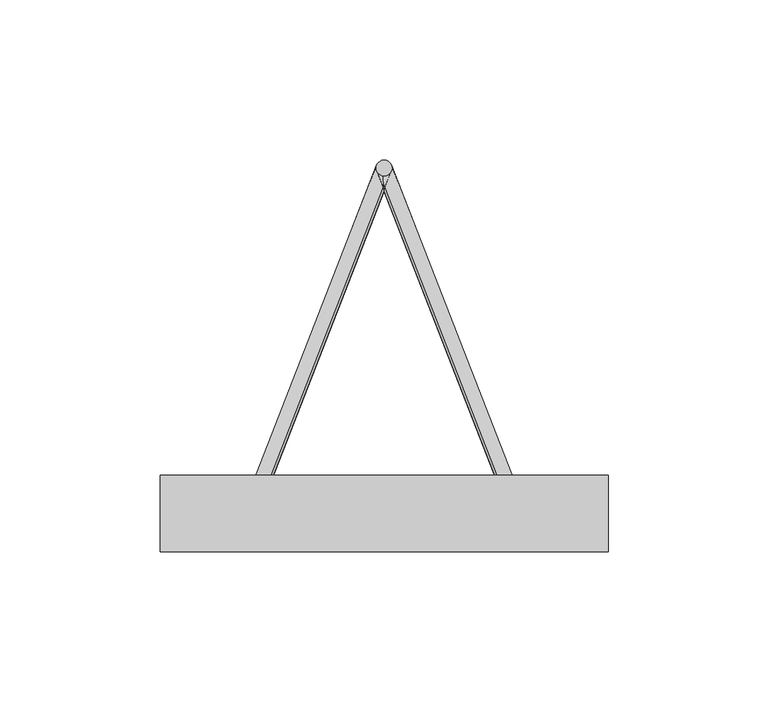
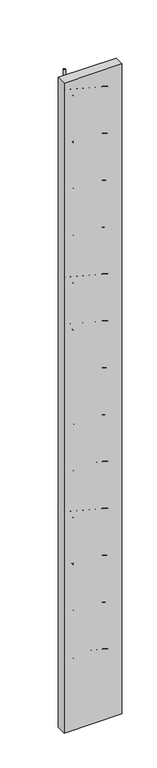
"""IFC4 building model written with IfcOpenShell, lengths in millimetres: proxy geometry, Vigota 2 (Pano 8) (Mf = 158)."""

from ifc_helpers import new_model, si_unit, point, frame, frame_2d, origin, origin_with_axes, origin_2d, place, context, project, spatial, polyline, circle_curve, trimmed, segment, composite_curve, outline, extrude, source, transform, mapped, element, save


def structural_framing_ade8639b(model_context):
    return source(origin(), model_context, "Body", "SweptSolid", [
        extrude(outline(polyline([(-70.0, 12.0), (70.0, 12.0), (70.0, -12.0), (-70.0, -12.0), (-70.0, 12.0)])), origin_with_axes(), (0.0, 0.0, 1.0), 1663.655183),
        extrude(outline(composite_curve([segment(trimmed(circle_curve(frame_2d((42.0, 0.0)), 2.5), [point((44.5, 0.0))], [point((39.5, 0.0))], False, "CARTESIAN"), True, "CONTINUOUS"), segment(trimmed(circle_curve(frame_2d((42.0, 0.0)), 2.5), [point((39.5, 0.0))], [point((44.5, 0.0))], False, "CARTESIAN"), True, "CONTINUOUS")], self_intersect=False)), frame((0.0, 0.0, 28.0), z_axis=(0.0, 0.0, 1.0), x_axis=(1.0, 0.0, 0.0)), (0.0, 0.0, 1.0), 1607.655183),
        extrude(outline(composite_curve([segment(trimmed(circle_curve(frame_2d((0.0, 108.0)), 2.5), [point((2.5, 108.0))], [point((-2.5, 108.0))], False, "CARTESIAN"), True, "CONTINUOUS"), segment(trimmed(circle_curve(frame_2d((0.0, 108.0)), 2.5), [point((-2.5, 108.0))], [point((2.5, 108.0))], False, "CARTESIAN"), True, "CONTINUOUS")], self_intersect=False)), frame((0.0, 0.0, 61.8275917), z_axis=(0.0, 0.0, 1.0), x_axis=(1.0, 0.0, 0.0)), (0.0, 0.0, 1.0), 1540.0),
        extrude(outline(composite_curve([segment(trimmed(circle_curve(origin_2d(), 2.5), [point((2.5, 0.0))], [point((-2.5, 0.0))], False, "CARTESIAN"), True, "CONTINUOUS"), segment(trimmed(circle_curve(origin_2d(), 2.5), [point((-2.5, 0.0))], [point((2.5, 0.0))], False, "CARTESIAN"), True, "CONTINUOUS")], self_intersect=False)), frame((42.0, 0.0, 51.8275917), z_axis=(-0.3218603428886276, 0.8276408817707567, 0.4598004898837537), x_axis=(0.8192319205108605, -3.936835275445103e-11, 0.5734623443750141)), (0.0, 0.0, 1.0), 130.491379),
        extrude(outline(composite_curve([segment(trimmed(circle_curve(origin_2d(), 2.5), [point((2.5, 0.0))], [point((-2.5, 0.0))], False, "CARTESIAN"), True, "CONTINUOUS"), segment(trimmed(circle_curve(origin_2d(), 2.5), [point((-2.5, 0.0))], [point((2.5, 0.0))], False, "CARTESIAN"), True, "CONTINUOUS")], self_intersect=False)), frame((0.0, 108.0, 111.8275917), z_axis=(0.3218603428886276, -0.8276408817707567, 0.4598004898837537), x_axis=(0.8192319205108605, -3.936835275445103e-11, -0.5734623443750141)), (0.0, 0.0, 1.0), 130.491379),
        extrude(outline(composite_curve([segment(trimmed(circle_curve(origin_2d(), 2.5), [point((2.5, 0.0))], [point((-2.5, 0.0))], False, "CARTESIAN"), True, "CONTINUOUS"), segment(trimmed(circle_curve(origin_2d(), 2.5), [point((-2.5, 0.0))], [point((2.5, 0.0))], False, "CARTESIAN"), True, "CONTINUOUS")], self_intersect=False)), frame((42.0, 0.0, 171.8275917), z_axis=(-0.3218603428886276, 0.8276408817707567, 0.4598004898837537), x_axis=(0.8192319205108605, -3.936835275445103e-11, 0.5734623443750141)), (0.0, 0.0, 1.0), 130.491379),
        extrude(outline(composite_curve([segment(trimmed(circle_curve(origin_2d(), 2.5), [point((2.5, 0.0))], [point((-2.5, 0.0))], False, "CARTESIAN"), True, "CONTINUOUS"), segment(trimmed(circle_curve(origin_2d(), 2.5), [point((-2.5, 0.0))], [point((2.5, 0.0))], False, "CARTESIAN"), True, "CONTINUOUS")], self_intersect=False)), frame((0.0, 108.0, 231.8275917), z_axis=(0.3218603428886276, -0.8276408817707567, 0.4598004898837537), x_axis=(0.8192319205108605, -3.936835275445103e-11, -0.5734623443750141)), (0.0, 0.0, 1.0), 130.491379),
        extrude(outline(composite_curve([segment(trimmed(circle_curve(origin_2d(), 2.5), [point((2.5, 0.0))], [point((-2.5, 0.0))], False, "CARTESIAN"), True, "CONTINUOUS"), segment(trimmed(circle_curve(origin_2d(), 2.5), [point((-2.5, 0.0))], [point((2.5, 0.0))], False, "CARTESIAN"), True, "CONTINUOUS")], self_intersect=False)), frame((42.0, 0.0, 291.8275917), z_axis=(-0.3218603428886276, 0.8276408817707567, 0.4598004898837537), x_axis=(0.8192319205108605, -3.936835275445103e-11, 0.5734623443750141)), (0.0, 0.0, 1.0), 130.491379),
        extrude(outline(composite_curve([segment(trimmed(circle_curve(origin_2d(), 2.5), [point((2.5, 0.0))], [point((-2.5, 0.0))], False, "CARTESIAN"), True, "CONTINUOUS"), segment(trimmed(circle_curve(origin_2d(), 2.5), [point((-2.5, 0.0))], [point((2.5, 0.0))], False, "CARTESIAN"), True, "CONTINUOUS")], self_intersect=False)), frame((0.0, 108.0, 351.8275917), z_axis=(0.3218603428886276, -0.8276408817707567, 0.4598004898837537), x_axis=(0.8192319205108605, -3.936835275445103e-11, -0.5734623443750141)), (0.0, 0.0, 1.0), 130.491379),
        extrude(outline(composite_curve([segment(trimmed(circle_curve(origin_2d(), 2.5), [point((2.5, 0.0))], [point((-2.5, 0.0))], False, "CARTESIAN"), True, "CONTINUOUS"), segment(trimmed(circle_curve(origin_2d(), 2.5), [point((-2.5, 0.0))], [point((2.5, 0.0))], False, "CARTESIAN"), True, "CONTINUOUS")], self_intersect=False)), frame((42.0, 0.0, 411.8275917), z_axis=(-0.3218603428886276, 0.8276408817707567, 0.4598004898837537), x_axis=(0.8192319205108605, -3.936835275445103e-11, 0.5734623443750141)), (0.0, 0.0, 1.0), 130.491379),
        extrude(outline(composite_curve([segment(trimmed(circle_curve(origin_2d(), 2.5), [point((2.5, 0.0))], [point((-2.5, 0.0))], False, "CARTESIAN"), True, "CONTINUOUS"), segment(trimmed(circle_curve(origin_2d(), 2.5), [point((-2.5, 0.0))], [point((2.5, 0.0))], False, "CARTESIAN"), True, "CONTINUOUS")], self_intersect=False)), frame((0.0, 108.0, 471.8275917), z_axis=(0.3218603428886276, -0.8276408817707567, 0.4598004898837537), x_axis=(0.8192319205108605, -3.936835275445103e-11, -0.5734623443750141)), (0.0, 0.0, 1.0), 130.491379),
        extrude(outline(composite_curve([segment(trimmed(circle_curve(origin_2d(), 2.5), [point((2.5, 0.0))], [point((-2.5, 0.0))], False, "CARTESIAN"), True, "CONTINUOUS"), segment(trimmed(circle_curve(origin_2d(), 2.5), [point((-2.5, 0.0))], [point((2.5, 0.0))], False, "CARTESIAN"), True, "CONTINUOUS")], self_intersect=False)), frame((42.0, 0.0, 531.8275917), z_axis=(-0.3218603428886276, 0.8276408817707567, 0.4598004898837537), x_axis=(0.8192319205108605, -3.936835275445103e-11, 0.5734623443750141)), (0.0, 0.0, 1.0), 130.491379),
        extrude(outline(composite_curve([segment(trimmed(circle_curve(origin_2d(), 2.5), [point((2.5, 0.0))], [point((-2.5, 0.0))], False, "CARTESIAN"), True, "CONTINUOUS"), segment(trimmed(circle_curve(origin_2d(), 2.5), [point((-2.5, 0.0))], [point((2.5, 0.0))], False, "CARTESIAN"), True, "CONTINUOUS")], self_intersect=False)), frame((0.0, 108.0, 591.8275917), z_axis=(0.3218603428886276, -0.8276408817707567, 0.4598004898837537), x_axis=(0.8192319205108605, -3.936835275445103e-11, -0.5734623443750141)), (0.0, 0.0, 1.0), 130.491379),
        extrude(outline(composite_curve([segment(trimmed(circle_curve(origin_2d(), 2.5), [point((2.5, 0.0))], [point((-2.5, 0.0))], False, "CARTESIAN"), True, "CONTINUOUS"), segment(trimmed(circle_curve(origin_2d(), 2.5), [point((-2.5, 0.0))], [point((2.5, 0.0))], False, "CARTESIAN"), True, "CONTINUOUS")], self_intersect=False)), frame((42.0, 0.0, 651.8275917), z_axis=(-0.3218603428886276, 0.8276408817707567, 0.4598004898837537), x_axis=(0.8192319205108605, -3.936835275445103e-11, 0.5734623443750141)), (0.0, 0.0, 1.0), 130.491379),
        extrude(outline(composite_curve([segment(trimmed(circle_curve(origin_2d(), 2.5), [point((2.5, 0.0))], [point((-2.5, 0.0))], False, "CARTESIAN"), True, "CONTINUOUS"), segment(trimmed(circle_curve(origin_2d(), 2.5), [point((-2.5, 0.0))], [point((2.5, 0.0))], False, "CARTESIAN"), True, "CONTINUOUS")], self_intersect=False)), frame((0.0, 108.0, 711.8275917), z_axis=(0.3218603428886276, -0.8276408817707567, 0.4598004898837537), x_axis=(0.8192319205108605, -3.936835275445103e-11, -0.5734623443750141)), (0.0, 0.0, 1.0), 130.491379),
        extrude(outline(composite_curve([segment(trimmed(circle_curve(origin_2d(), 2.5), [point((2.5, 0.0))], [point((-2.5, 0.0))], False, "CARTESIAN"), True, "CONTINUOUS"), segment(trimmed(circle_curve(origin_2d(), 2.5), [point((-2.5, 0.0))], [point((2.5, 0.0))], False, "CARTESIAN"), True, "CONTINUOUS")], self_intersect=False)), frame((42.0, 0.0, 771.8275917), z_axis=(-0.3218603428886276, 0.8276408817707567, 0.4598004898837537), x_axis=(0.8192319205108605, -3.936835275445103e-11, 0.5734623443750141)), (0.0, 0.0, 1.0), 130.491379),
        extrude(outline(composite_curve([segment(trimmed(circle_curve(origin_2d(), 2.5), [point((2.5, 0.0))], [point((-2.5, 0.0))], False, "CARTESIAN"), True, "CONTINUOUS"), segment(trimmed(circle_curve(origin_2d(), 2.5), [point((-2.5, 0.0))], [point((2.5, 0.0))], False, "CARTESIAN"), True, "CONTINUOUS")], self_intersect=False)), frame((0.0, 108.0, 831.8275917), z_axis=(0.3218603428886276, -0.8276408817707567, 0.4598004898837537), x_axis=(0.8192319205108605, -3.936835275445103e-11, -0.5734623443750141)), (0.0, 0.0, 1.0), 130.491379),
        extrude(outline(composite_curve([segment(trimmed(circle_curve(origin_2d(), 2.5), [point((2.5, 0.0))], [point((-2.5, 0.0))], False, "CARTESIAN"), True, "CONTINUOUS"), segment(trimmed(circle_curve(origin_2d(), 2.5), [point((-2.5, 0.0))], [point((2.5, 0.0))], False, "CARTESIAN"), True, "CONTINUOUS")], self_intersect=False)), frame((42.0, 0.0, 891.8275917), z_axis=(-0.3218603428886276, 0.8276408817707567, 0.4598004898837537), x_axis=(0.8192319205108605, -3.936835275445103e-11, 0.5734623443750141)), (0.0, 0.0, 1.0), 130.491379),
        extrude(outline(composite_curve([segment(trimmed(circle_curve(origin_2d(), 2.5), [point((2.5, 0.0))], [point((-2.5, 0.0))], False, "CARTESIAN"), True, "CONTINUOUS"), segment(trimmed(circle_curve(origin_2d(), 2.5), [point((-2.5, 0.0))], [point((2.5, 0.0))], False, "CARTESIAN"), True, "CONTINUOUS")], self_intersect=False)), frame((0.0, 108.0, 951.8275917), z_axis=(0.3218603428886276, -0.8276408817707567, 0.4598004898837537), x_axis=(0.8192319205108605, -3.936835275445103e-11, -0.5734623443750141)), (0.0, 0.0, 1.0), 130.491379),
        extrude(outline(composite_curve([segment(trimmed(circle_curve(origin_2d(), 2.5), [point((2.5, 0.0))], [point((-2.5, 0.0))], False, "CARTESIAN"), True, "CONTINUOUS"), segment(trimmed(circle_curve(origin_2d(), 2.5), [point((-2.5, 0.0))], [point((2.5, 0.0))], False, "CARTESIAN"), True, "CONTINUOUS")], self_intersect=False)), frame((42.0, 0.0, 1011.8275917), z_axis=(-0.3218603428886276, 0.8276408817707567, 0.4598004898837537), x_axis=(0.8192319205108605, -3.936835275445103e-11, 0.5734623443750141)), (0.0, 0.0, 1.0), 130.491379),
        extrude(outline(composite_curve([segment(trimmed(circle_curve(origin_2d(), 2.5), [point((2.5, 0.0))], [point((-2.5, 0.0))], False, "CARTESIAN"), True, "CONTINUOUS"), segment(trimmed(circle_curve(origin_2d(), 2.5), [point((-2.5, 0.0))], [point((2.5, 0.0))], False, "CARTESIAN"), True, "CONTINUOUS")], self_intersect=False)), frame((0.0, 108.0, 1071.827592), z_axis=(0.3218603428886276, -0.8276408817707567, 0.4598004898837537), x_axis=(0.8192319205108605, -3.936835275445103e-11, -0.5734623443750141)), (0.0, 0.0, 1.0), 130.491379),
        extrude(outline(composite_curve([segment(trimmed(circle_curve(origin_2d(), 2.5), [point((2.5, 0.0))], [point((-2.5, 0.0))], False, "CARTESIAN"), True, "CONTINUOUS"), segment(trimmed(circle_curve(origin_2d(), 2.5), [point((-2.5, 0.0))], [point((2.5, 0.0))], False, "CARTESIAN"), True, "CONTINUOUS")], self_intersect=False)), frame((42.0, 0.0, 1131.827592), z_axis=(-0.3218603428886276, 0.8276408817707567, 0.4598004898837537), x_axis=(0.8192319205108605, -3.936835275445103e-11, 0.5734623443750141)), (0.0, 0.0, 1.0), 130.491379),
        extrude(outline(composite_curve([segment(trimmed(circle_curve(origin_2d(), 2.5), [point((2.5, 0.0))], [point((-2.5, 0.0))], False, "CARTESIAN"), True, "CONTINUOUS"), segment(trimmed(circle_curve(origin_2d(), 2.5), [point((-2.5, 0.0))], [point((2.5, 0.0))], False, "CARTESIAN"), True, "CONTINUOUS")], self_intersect=False)), frame((0.0, 108.0, 1191.827592), z_axis=(0.3218603428886276, -0.8276408817707567, 0.4598004898837537), x_axis=(0.8192319205108605, -3.936835275445103e-11, -0.5734623443750141)), (0.0, 0.0, 1.0), 130.491379),
        extrude(outline(composite_curve([segment(trimmed(circle_curve(origin_2d(), 2.5), [point((2.5, 0.0))], [point((-2.5, 0.0))], False, "CARTESIAN"), True, "CONTINUOUS"), segment(trimmed(circle_curve(origin_2d(), 2.5), [point((-2.5, 0.0))], [point((2.5, 0.0))], False, "CARTESIAN"), True, "CONTINUOUS")], self_intersect=False)), frame((42.0, 0.0, 1251.827592), z_axis=(-0.3218603428886276, 0.8276408817707567, 0.4598004898837537), x_axis=(0.8192319205108605, -3.936835275445103e-11, 0.5734623443750141)), (0.0, 0.0, 1.0), 130.491379),
        extrude(outline(composite_curve([segment(trimmed(circle_curve(origin_2d(), 2.5), [point((2.5, 0.0))], [point((-2.5, 0.0))], False, "CARTESIAN"), True, "CONTINUOUS"), segment(trimmed(circle_curve(origin_2d(), 2.5), [point((-2.5, 0.0))], [point((2.5, 0.0))], False, "CARTESIAN"), True, "CONTINUOUS")], self_intersect=False)), frame((0.0, 108.0, 1311.827592), z_axis=(0.3218603428886276, -0.8276408817707567, 0.4598004898837537), x_axis=(0.8192319205108605, -3.936835275445103e-11, -0.5734623443750141)), (0.0, 0.0, 1.0), 130.491379),
        extrude(outline(composite_curve([segment(trimmed(circle_curve(origin_2d(), 2.5), [point((2.5, 0.0))], [point((-2.5, 0.0))], False, "CARTESIAN"), True, "CONTINUOUS"), segment(trimmed(circle_curve(origin_2d(), 2.5), [point((-2.5, 0.0))], [point((2.5, 0.0))], False, "CARTESIAN"), True, "CONTINUOUS")], self_intersect=False)), frame((42.0, 0.0, 1371.827592), z_axis=(-0.3218603428886276, 0.8276408817707567, 0.4598004898837537), x_axis=(0.8192319205108605, -3.936835275445103e-11, 0.5734623443750141)), (0.0, 0.0, 1.0), 130.491379),
        extrude(outline(composite_curve([segment(trimmed(circle_curve(origin_2d(), 2.5), [point((2.5, 0.0))], [point((-2.5, 0.0))], False, "CARTESIAN"), True, "CONTINUOUS"), segment(trimmed(circle_curve(origin_2d(), 2.5), [point((-2.5, 0.0))], [point((2.5, 0.0))], False, "CARTESIAN"), True, "CONTINUOUS")], self_intersect=False)), frame((0.0, 108.0, 1431.827592), z_axis=(0.3218603428886276, -0.8276408817707567, 0.4598004898837537), x_axis=(0.8192319205108605, -3.936835275445103e-11, -0.5734623443750141)), (0.0, 0.0, 1.0), 130.491379),
        extrude(outline(composite_curve([segment(trimmed(circle_curve(origin_2d(), 2.5), [point((2.5, 0.0))], [point((-2.5, 0.0))], False, "CARTESIAN"), True, "CONTINUOUS"), segment(trimmed(circle_curve(origin_2d(), 2.5), [point((-2.5, 0.0))], [point((2.5, 0.0))], False, "CARTESIAN"), True, "CONTINUOUS")], self_intersect=False)), frame((42.0, 0.0, 1491.827592), z_axis=(-0.3218603428886276, 0.8276408817707567, 0.4598004898837537), x_axis=(0.8192319205108605, -3.936835275445103e-11, 0.5734623443750141)), (0.0, 0.0, 1.0), 130.491379),
        extrude(outline(composite_curve([segment(trimmed(circle_curve(origin_2d(), 2.5), [point((2.5, 0.0))], [point((-2.5, 0.0))], False, "CARTESIAN"), True, "CONTINUOUS"), segment(trimmed(circle_curve(origin_2d(), 2.5), [point((-2.5, 0.0))], [point((2.5, 0.0))], False, "CARTESIAN"), True, "CONTINUOUS")], self_intersect=False)), frame((0.0, 108.0, 1551.827592), z_axis=(0.3218603428886276, -0.8276408817707567, 0.4598004898837537), x_axis=(0.8192319205108605, -3.936835275445103e-11, -0.5734623443750141)), (0.0, 0.0, 1.0), 130.491379),
        extrude(outline(composite_curve([segment(trimmed(circle_curve(frame_2d((-42.0, 0.0)), 2.5), [point((-39.5, 0.0))], [point((-44.5, 0.0))], False, "CARTESIAN"), True, "CONTINUOUS"), segment(trimmed(circle_curve(frame_2d((-42.0, 0.0)), 2.5), [point((-44.5, 0.0))], [point((-39.5, 0.0))], False, "CARTESIAN"), True, "CONTINUOUS")], self_intersect=False)), frame((0.0, 0.0, 28.0), z_axis=(0.0, 0.0, 1.0), x_axis=(1.0, 0.0, 0.0)), (0.0, 0.0, 1.0), 1607.655183),
        extrude(outline(composite_curve([segment(trimmed(circle_curve(origin_2d(), 2.5), [point((2.5, 0.0))], [point((-2.5, 0.0))], False, "CARTESIAN"), True, "CONTINUOUS"), segment(trimmed(circle_curve(origin_2d(), 2.5), [point((-2.5, 0.0))], [point((2.5, 0.0))], False, "CARTESIAN"), True, "CONTINUOUS")], self_intersect=False)), frame((-42.0, 0.0, 51.8275917), z_axis=(0.3218603428886276, 0.8276408817707567, 0.4598004898837537), x_axis=(0.8192319205108605, 3.936835275445103e-11, -0.5734623443750141)), (0.0, 0.0, 1.0), 130.491379),
        extrude(outline(composite_curve([segment(trimmed(circle_curve(origin_2d(), 2.5), [point((2.5, 0.0))], [point((-2.5, 0.0))], False, "CARTESIAN"), True, "CONTINUOUS"), segment(trimmed(circle_curve(origin_2d(), 2.5), [point((-2.5, 0.0))], [point((2.5, 0.0))], False, "CARTESIAN"), True, "CONTINUOUS")], self_intersect=False)), frame((0.0, 108.0, 111.8275917), z_axis=(-0.3218603428886276, -0.8276408817707567, 0.4598004898837537), x_axis=(0.8192319205108605, 3.936835275445103e-11, 0.5734623443750141)), (0.0, 0.0, 1.0), 130.491379),
        extrude(outline(composite_curve([segment(trimmed(circle_curve(origin_2d(), 2.5), [point((2.5, 0.0))], [point((-2.5, 0.0))], False, "CARTESIAN"), True, "CONTINUOUS"), segment(trimmed(circle_curve(origin_2d(), 2.5), [point((-2.5, 0.0))], [point((2.5, 0.0))], False, "CARTESIAN"), True, "CONTINUOUS")], self_intersect=False)), frame((-42.0, 0.0, 171.8275917), z_axis=(0.3218603428886276, 0.8276408817707567, 0.4598004898837537), x_axis=(0.8192319205108605, 3.936835275445103e-11, -0.5734623443750141)), (0.0, 0.0, 1.0), 130.491379),
        extrude(outline(composite_curve([segment(trimmed(circle_curve(origin_2d(), 2.5), [point((2.5, 0.0))], [point((-2.5, 0.0))], False, "CARTESIAN"), True, "CONTINUOUS"), segment(trimmed(circle_curve(origin_2d(), 2.5), [point((-2.5, 0.0))], [point((2.5, 0.0))], False, "CARTESIAN"), True, "CONTINUOUS")], self_intersect=False)), frame((0.0, 108.0, 231.8275917), z_axis=(-0.3218603428886276, -0.8276408817707567, 0.4598004898837537), x_axis=(0.8192319205108605, 3.936835275445103e-11, 0.5734623443750141)), (0.0, 0.0, 1.0), 130.491379),
        extrude(outline(composite_curve([segment(trimmed(circle_curve(origin_2d(), 2.5), [point((2.5, 0.0))], [point((-2.5, 0.0))], False, "CARTESIAN"), True, "CONTINUOUS"), segment(trimmed(circle_curve(origin_2d(), 2.5), [point((-2.5, 0.0))], [point((2.5, 0.0))], False, "CARTESIAN"), True, "CONTINUOUS")], self_intersect=False)), frame((-42.0, 0.0, 291.8275917), z_axis=(0.3218603428886276, 0.8276408817707567, 0.4598004898837537), x_axis=(0.8192319205108605, 3.936835275445103e-11, -0.5734623443750141)), (0.0, 0.0, 1.0), 130.491379),
        extrude(outline(composite_curve([segment(trimmed(circle_curve(origin_2d(), 2.5), [point((2.5, 0.0))], [point((-2.5, 0.0))], False, "CARTESIAN"), True, "CONTINUOUS"), segment(trimmed(circle_curve(origin_2d(), 2.5), [point((-2.5, 0.0))], [point((2.5, 0.0))], False, "CARTESIAN"), True, "CONTINUOUS")], self_intersect=False)), frame((0.0, 108.0, 351.8275917), z_axis=(-0.3218603428886276, -0.8276408817707567, 0.4598004898837537), x_axis=(0.8192319205108605, 3.936835275445103e-11, 0.5734623443750141)), (0.0, 0.0, 1.0), 130.491379),
        extrude(outline(composite_curve([segment(trimmed(circle_curve(origin_2d(), 2.5), [point((2.5, 0.0))], [point((-2.5, 0.0))], False, "CARTESIAN"), True, "CONTINUOUS"), segment(trimmed(circle_curve(origin_2d(), 2.5), [point((-2.5, 0.0))], [point((2.5, 0.0))], False, "CARTESIAN"), True, "CONTINUOUS")], self_intersect=False)), frame((-42.0, 0.0, 411.8275917), z_axis=(0.3218603428886276, 0.8276408817707567, 0.4598004898837537), x_axis=(0.8192319205108605, 3.936835275445103e-11, -0.5734623443750141)), (0.0, 0.0, 1.0), 130.491379),
        extrude(outline(composite_curve([segment(trimmed(circle_curve(origin_2d(), 2.5), [point((2.5, 0.0))], [point((-2.5, 0.0))], False, "CARTESIAN"), True, "CONTINUOUS"), segment(trimmed(circle_curve(origin_2d(), 2.5), [point((-2.5, 0.0))], [point((2.5, 0.0))], False, "CARTESIAN"), True, "CONTINUOUS")], self_intersect=False)), frame((0.0, 108.0, 471.8275917), z_axis=(-0.3218603428886276, -0.8276408817707567, 0.4598004898837537), x_axis=(0.8192319205108605, 3.936835275445103e-11, 0.5734623443750141)), (0.0, 0.0, 1.0), 130.491379),
        extrude(outline(composite_curve([segment(trimmed(circle_curve(origin_2d(), 2.5), [point((2.5, 0.0))], [point((-2.5, 0.0))], False, "CARTESIAN"), True, "CONTINUOUS"), segment(trimmed(circle_curve(origin_2d(), 2.5), [point((-2.5, 0.0))], [point((2.5, 0.0))], False, "CARTESIAN"), True, "CONTINUOUS")], self_intersect=False)), frame((-42.0, 0.0, 531.8275917), z_axis=(0.3218603428886276, 0.8276408817707567, 0.4598004898837537), x_axis=(0.8192319205108605, 3.936835275445103e-11, -0.5734623443750141)), (0.0, 0.0, 1.0), 130.491379),
        extrude(outline(composite_curve([segment(trimmed(circle_curve(origin_2d(), 2.5), [point((2.5, 0.0))], [point((-2.5, 0.0))], False, "CARTESIAN"), True, "CONTINUOUS"), segment(trimmed(circle_curve(origin_2d(), 2.5), [point((-2.5, 0.0))], [point((2.5, 0.0))], False, "CARTESIAN"), True, "CONTINUOUS")], self_intersect=False)), frame((0.0, 108.0, 591.8275917), z_axis=(-0.3218603428886276, -0.8276408817707567, 0.4598004898837537), x_axis=(0.8192319205108605, 3.936835275445103e-11, 0.5734623443750141)), (0.0, 0.0, 1.0), 130.491379),
        extrude(outline(composite_curve([segment(trimmed(circle_curve(origin_2d(), 2.5), [point((2.5, 0.0))], [point((-2.5, 0.0))], False, "CARTESIAN"), True, "CONTINUOUS"), segment(trimmed(circle_curve(origin_2d(), 2.5), [point((-2.5, 0.0))], [point((2.5, 0.0))], False, "CARTESIAN"), True, "CONTINUOUS")], self_intersect=False)), frame((-42.0, 0.0, 651.8275917), z_axis=(0.3218603428886276, 0.8276408817707567, 0.4598004898837537), x_axis=(0.8192319205108605, 3.936835275445103e-11, -0.5734623443750141)), (0.0, 0.0, 1.0), 130.491379),
        extrude(outline(composite_curve([segment(trimmed(circle_curve(origin_2d(), 2.5), [point((2.5, 0.0))], [point((-2.5, 0.0))], False, "CARTESIAN"), True, "CONTINUOUS"), segment(trimmed(circle_curve(origin_2d(), 2.5), [point((-2.5, 0.0))], [point((2.5, 0.0))], False, "CARTESIAN"), True, "CONTINUOUS")], self_intersect=False)), frame((0.0, 108.0, 711.8275917), z_axis=(-0.3218603428886276, -0.8276408817707567, 0.4598004898837537), x_axis=(0.8192319205108605, 3.936835275445103e-11, 0.5734623443750141)), (0.0, 0.0, 1.0), 130.491379),
        extrude(outline(composite_curve([segment(trimmed(circle_curve(origin_2d(), 2.5), [point((2.5, 0.0))], [point((-2.5, 0.0))], False, "CARTESIAN"), True, "CONTINUOUS"), segment(trimmed(circle_curve(origin_2d(), 2.5), [point((-2.5, 0.0))], [point((2.5, 0.0))], False, "CARTESIAN"), True, "CONTINUOUS")], self_intersect=False)), frame((-42.0, 0.0, 771.8275917), z_axis=(0.3218603428886276, 0.8276408817707567, 0.4598004898837537), x_axis=(0.8192319205108605, 3.936835275445103e-11, -0.5734623443750141)), (0.0, 0.0, 1.0), 130.491379),
        extrude(outline(composite_curve([segment(trimmed(circle_curve(origin_2d(), 2.5), [point((2.5, 0.0))], [point((-2.5, 0.0))], False, "CARTESIAN"), True, "CONTINUOUS"), segment(trimmed(circle_curve(origin_2d(), 2.5), [point((-2.5, 0.0))], [point((2.5, 0.0))], False, "CARTESIAN"), True, "CONTINUOUS")], self_intersect=False)), frame((0.0, 108.0, 831.8275917), z_axis=(-0.3218603428886276, -0.8276408817707567, 0.4598004898837537), x_axis=(0.8192319205108605, 3.936835275445103e-11, 0.5734623443750141)), (0.0, 0.0, 1.0), 130.491379),
        extrude(outline(composite_curve([segment(trimmed(circle_curve(origin_2d(), 2.5), [point((2.5, 0.0))], [point((-2.5, 0.0))], False, "CARTESIAN"), True, "CONTINUOUS"), segment(trimmed(circle_curve(origin_2d(), 2.5), [point((-2.5, 0.0))], [point((2.5, 0.0))], False, "CARTESIAN"), True, "CONTINUOUS")], self_intersect=False)), frame((-42.0, 0.0, 891.8275917), z_axis=(0.3218603428886276, 0.8276408817707567, 0.4598004898837537), x_axis=(0.8192319205108605, 3.936835275445103e-11, -0.5734623443750141)), (0.0, 0.0, 1.0), 130.491379),
        extrude(outline(composite_curve([segment(trimmed(circle_curve(origin_2d(), 2.5), [point((2.5, 0.0))], [point((-2.5, 0.0))], False, "CARTESIAN"), True, "CONTINUOUS"), segment(trimmed(circle_curve(origin_2d(), 2.5), [point((-2.5, 0.0))], [point((2.5, 0.0))], False, "CARTESIAN"), True, "CONTINUOUS")], self_intersect=False)), frame((0.0, 108.0, 951.8275917), z_axis=(-0.3218603428886276, -0.8276408817707567, 0.4598004898837537), x_axis=(0.8192319205108605, 3.936835275445103e-11, 0.5734623443750141)), (0.0, 0.0, 1.0), 130.491379),
        extrude(outline(composite_curve([segment(trimmed(circle_curve(origin_2d(), 2.5), [point((2.5, 0.0))], [point((-2.5, 0.0))], False, "CARTESIAN"), True, "CONTINUOUS"), segment(trimmed(circle_curve(origin_2d(), 2.5), [point((-2.5, 0.0))], [point((2.5, 0.0))], False, "CARTESIAN"), True, "CONTINUOUS")], self_intersect=False)), frame((-42.0, 0.0, 1011.8275917), z_axis=(0.3218603428886276, 0.8276408817707567, 0.4598004898837537), x_axis=(0.8192319205108605, 3.936835275445103e-11, -0.5734623443750141)), (0.0, 0.0, 1.0), 130.491379),
        extrude(outline(composite_curve([segment(trimmed(circle_curve(origin_2d(), 2.5), [point((2.5, 0.0))], [point((-2.5, 0.0))], False, "CARTESIAN"), True, "CONTINUOUS"), segment(trimmed(circle_curve(origin_2d(), 2.5), [point((-2.5, 0.0))], [point((2.5, 0.0))], False, "CARTESIAN"), True, "CONTINUOUS")], self_intersect=False)), frame((0.0, 108.0, 1071.827592), z_axis=(-0.3218603428886276, -0.8276408817707567, 0.4598004898837537), x_axis=(0.8192319205108605, 3.936835275445103e-11, 0.5734623443750141)), (0.0, 0.0, 1.0), 130.491379),
        extrude(outline(composite_curve([segment(trimmed(circle_curve(origin_2d(), 2.5), [point((2.5, 0.0))], [point((-2.5, 0.0))], False, "CARTESIAN"), True, "CONTINUOUS"), segment(trimmed(circle_curve(origin_2d(), 2.5), [point((-2.5, 0.0))], [point((2.5, 0.0))], False, "CARTESIAN"), True, "CONTINUOUS")], self_intersect=False)), frame((-42.0, 0.0, 1131.827592), z_axis=(0.3218603428886276, 0.8276408817707567, 0.4598004898837537), x_axis=(0.8192319205108605, 3.936835275445103e-11, -0.5734623443750141)), (0.0, 0.0, 1.0), 130.491379),
        extrude(outline(composite_curve([segment(trimmed(circle_curve(origin_2d(), 2.5), [point((2.5, 0.0))], [point((-2.5, 0.0))], False, "CARTESIAN"), True, "CONTINUOUS"), segment(trimmed(circle_curve(origin_2d(), 2.5), [point((-2.5, 0.0))], [point((2.5, 0.0))], False, "CARTESIAN"), True, "CONTINUOUS")], self_intersect=False)), frame((0.0, 108.0, 1191.827592), z_axis=(-0.3218603428886276, -0.8276408817707567, 0.4598004898837537), x_axis=(0.8192319205108605, 3.936835275445103e-11, 0.5734623443750141)), (0.0, 0.0, 1.0), 130.491379),
        extrude(outline(composite_curve([segment(trimmed(circle_curve(origin_2d(), 2.5), [point((2.5, 0.0))], [point((-2.5, 0.0))], False, "CARTESIAN"), True, "CONTINUOUS"), segment(trimmed(circle_curve(origin_2d(), 2.5), [point((-2.5, 0.0))], [point((2.5, 0.0))], False, "CARTESIAN"), True, "CONTINUOUS")], self_intersect=False)), frame((-42.0, 0.0, 1251.827592), z_axis=(0.3218603428886276, 0.8276408817707567, 0.4598004898837537), x_axis=(0.8192319205108605, 3.936835275445103e-11, -0.5734623443750141)), (0.0, 0.0, 1.0), 130.491379),
        extrude(outline(composite_curve([segment(trimmed(circle_curve(origin_2d(), 2.5), [point((2.5, 0.0))], [point((-2.5, 0.0))], False, "CARTESIAN"), True, "CONTINUOUS"), segment(trimmed(circle_curve(origin_2d(), 2.5), [point((-2.5, 0.0))], [point((2.5, 0.0))], False, "CARTESIAN"), True, "CONTINUOUS")], self_intersect=False)), frame((0.0, 108.0, 1311.827592), z_axis=(-0.3218603428886276, -0.8276408817707567, 0.4598004898837537), x_axis=(0.8192319205108605, 3.936835275445103e-11, 0.5734623443750141)), (0.0, 0.0, 1.0), 130.491379),
        extrude(outline(composite_curve([segment(trimmed(circle_curve(origin_2d(), 2.5), [point((2.5, 0.0))], [point((-2.5, 0.0))], False, "CARTESIAN"), True, "CONTINUOUS"), segment(trimmed(circle_curve(origin_2d(), 2.5), [point((-2.5, 0.0))], [point((2.5, 0.0))], False, "CARTESIAN"), True, "CONTINUOUS")], self_intersect=False)), frame((-42.0, 0.0, 1371.827592), z_axis=(0.3218603428886276, 0.8276408817707567, 0.4598004898837537), x_axis=(0.8192319205108605, 3.936835275445103e-11, -0.5734623443750141)), (0.0, 0.0, 1.0), 130.491379),
        extrude(outline(composite_curve([segment(trimmed(circle_curve(origin_2d(), 2.5), [point((2.5, 0.0))], [point((-2.5, 0.0))], False, "CARTESIAN"), True, "CONTINUOUS"), segment(trimmed(circle_curve(origin_2d(), 2.5), [point((-2.5, 0.0))], [point((2.5, 0.0))], False, "CARTESIAN"), True, "CONTINUOUS")], self_intersect=False)), frame((0.0, 108.0, 1431.827592), z_axis=(-0.3218603428886276, -0.8276408817707567, 0.4598004898837537), x_axis=(0.8192319205108605, 3.936835275445103e-11, 0.5734623443750141)), (0.0, 0.0, 1.0), 130.491379),
        extrude(outline(composite_curve([segment(trimmed(circle_curve(origin_2d(), 2.5), [point((2.5, 0.0))], [point((-2.5, 0.0))], False, "CARTESIAN"), True, "CONTINUOUS"), segment(trimmed(circle_curve(origin_2d(), 2.5), [point((-2.5, 0.0))], [point((2.5, 0.0))], False, "CARTESIAN"), True, "CONTINUOUS")], self_intersect=False)), frame((-42.0, 0.0, 1491.827592), z_axis=(0.3218603428886276, 0.8276408817707567, 0.4598004898837537), x_axis=(0.8192319205108605, 3.936835275445103e-11, -0.5734623443750141)), (0.0, 0.0, 1.0), 130.491379),
        extrude(outline(composite_curve([segment(trimmed(circle_curve(origin_2d(), 2.5), [point((2.5, 0.0))], [point((-2.5, 0.0))], False, "CARTESIAN"), True, "CONTINUOUS"), segment(trimmed(circle_curve(origin_2d(), 2.5), [point((-2.5, 0.0))], [point((2.5, 0.0))], False, "CARTESIAN"), True, "CONTINUOUS")], self_intersect=False)), frame((0.0, 108.0, 1551.827592), z_axis=(-0.3218603428886276, -0.8276408817707567, 0.4598004898837537), x_axis=(0.8192319205108605, 3.936835275445103e-11, 0.5734623443750141)), (0.0, 0.0, 1.0), 130.491379),
    ])


if __name__ == "__main__":
    model = new_model("IFC4")
    model_context = context("Model", 3, world=origin())
    ifc_project = project(units=[si_unit("LENGTHUNIT", "METRE", prefix="MILLI")], contexts=[model_context])
    site = spatial("IfcSite", under=ifc_project)
    building = spatial("IfcBuilding", under=site)
    placement = place(None, origin())
    structural_framing_shape = structural_framing_ade8639b(model_context)
    element("IfcBuildingElementProxy", 1, Name="Vigota 2 (Pano 8) (Mf = 158)", ObjectType="Vigota 2 (Pano 8) (Mf = 158)", at=placement, inside=building, context=model_context, shape_type="MappedRepresentation", body=[
        mapped(structural_framing_shape, transform((0.0, 0.0, 0.0), x_axis=(1.0, 0.0, 0.0), y_axis=(0.0, 1.0, 0.0), z_axis=(0.0, 0.0, 1.0))),
    ])
    save(model, "model.ifc")

# Revit data of these elements
# Element 1 (IfcBuildingElementProxy, "Vigota 2 (Pano 8) (Mf = 158)")
#   Materials on its faces: "Aço", "Concreto armado"
# Materials
#   "Aço": class "Metal", colour RGB 120 120 120, transparency 0, Description = "Aço estrutural A36 grau, ASTM B, acabamento laminado", Cost = 0
#   "Concreto armado": class "Não atribuído", colour RGB 168 169 158, transparency 0
